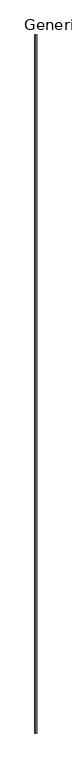
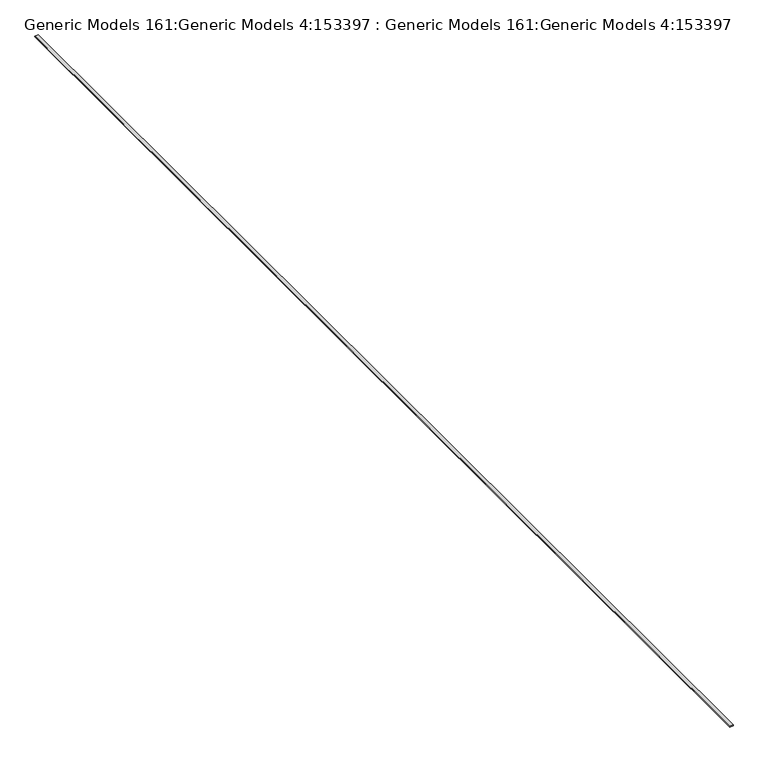
"""IFC4 building model written with IfcOpenShell, lengths in millimetres: proxy geometry, Generic Models 161:Generic Models 4:153397 : Generic Models 161:Generic Models 4:153397."""

import ifcopenshell
import ifcopenshell.guid

model = None  # the IFC model being written
_history = None  # IfcOwnerHistory: only IFC2X3 demands one
_inside = {}  # id of a spatial element -> (the spatial element, [elements in it])
_under = {}  # id of a project, library or spatial element -> (it, [spatial elements below it])
_declared = {}  # id of a project -> (the project, [libraries it declares])
_typed = {}  # id of a type object -> (the type object, [elements of that type])
_made_of = {}  # id of a material, layer set ... -> (it, [elements and type objects made of it])


def new_model(schema):
    """Start an empty IFC model of exactly this schema.

    Asked for "IFC4X3", IfcOpenShell would pick the latest addendum, in which some entities
    have other attributes; the version numbers below select the first issue.
    IFC2X3 requires an IfcOwnerHistory on every rooted entity: one is made here for all.
    """
    global model, _history
    if schema == "IFC4X3":
        model = ifcopenshell.file(schema_version=(4, 3, 0, 0))
    else:
        model = ifcopenshell.file(schema=schema)
    _inside.clear()
    _under.clear()
    _declared.clear()
    _typed.clear()
    _made_of.clear()
    _history = None
    if model.schema == "IFC2X3":
        org = make("IfcOrganization", Name="unknown")
        user = make(
            "IfcPersonAndOrganization",
            ThePerson=make("IfcPerson", FamilyName="unknown"),
            TheOrganization=org,
        )
        app = make(
            "IfcApplication",
            ApplicationDeveloper=org,
            Version="unknown",
            ApplicationFullName="unknown",
            ApplicationIdentifier="unknown",
        )
        _history = make(
            "IfcOwnerHistory",
            OwningUser=user,
            OwningApplication=app,
            ChangeAction="ADDED",
            CreationDate=0,
        )
    return model


def make(cls, **values):
    """One entity of the class cls with the attributes given. An attribute that is None is left unset."""
    return model.create_entity(
        cls, **{name: value for name, value in values.items() if value is not None}
    )


def rooted(cls, **values):
    """An entity with a GlobalId (a new one), such as an element, a storey or a relation."""
    return make(cls, GlobalId=ifcopenshell.guid.new(), OwnerHistory=_history, **values)


def si_unit(unit_type, name, prefix=None):
    """IfcSIUnit, for example si_unit("LENGTHUNIT", "METRE", prefix="MILLI")."""
    return make("IfcSIUnit", UnitType=unit_type, Prefix=prefix, Name=name)


def assignment(units):
    """IfcUnitAssignment: the units of a project."""
    return None if units is None else make("IfcUnitAssignment", Units=units)


def point(xyz):
    """IfcCartesianPoint."""
    return None if xyz is None else make("IfcCartesianPoint", Coordinates=xyz)


def direction(xyz):
    """IfcDirection."""
    return None if xyz is None else make("IfcDirection", DirectionRatios=xyz)


def frame(location, z_axis=None, x_axis=None):
    """IfcAxis2Placement3D, a coordinate frame: its origin and axes. An axis left out is left unset."""
    return make(
        "IfcAxis2Placement3D",
        Location=point(location),
        Axis=direction(z_axis),
        RefDirection=direction(x_axis),
    )


def frame_2d(location, x_axis=None):
    """IfcAxis2Placement2D, a coordinate frame in the plane: its origin and x axis."""
    return make(
        "IfcAxis2Placement2D", Location=point(location), RefDirection=direction(x_axis)
    )


def origin():
    """The frame at (0, 0, 0) with its axes left unset."""
    return frame((0.0, 0.0, 0.0))


def place(relative_to, where):
    """IfcLocalPlacement: puts the frame where relative to a parent placement (None: the world)."""
    return make(
        "IfcLocalPlacement", PlacementRelTo=relative_to, RelativePlacement=where
    )


def context(
    kind, dimensions, precision=None, world=None, true_north=None, identifier=None
):
    """IfcGeometricRepresentationContext, for example the 3D "Model" context."""
    return make(
        "IfcGeometricRepresentationContext",
        ContextIdentifier=identifier,
        ContextType=kind,
        CoordinateSpaceDimension=dimensions,
        Precision=precision,
        WorldCoordinateSystem=world,
        TrueNorth=true_north,
    )


def project(units=None, contexts=None):
    """IfcProject with its units and contexts."""
    return rooted(
        "IfcProject",
        Name="project",
        RepresentationContexts=contexts,
        UnitsInContext=assignment(units),
    )


def spatial(cls, under=None, at=None, **own):
    """A site, building, storey or space (cls), placed at a placement, below another one or the project."""
    s = rooted(cls, ObjectPlacement=at, **own)
    if under is not None:
        _under.setdefault(under.id(), (under, []))[1].append(s)
    return s


def polyline(points):
    """IfcPolyline through the points."""
    return make("IfcPolyline", Points=[point(p) for p in points])


def circle_curve(where, radius):
    """IfcCircle in the frame where."""
    return make("IfcCircle", Position=where, Radius=radius)


def trimmed(basis, trim1, trim2, sense, master):
    """IfcTrimmedCurve: the piece of a basis curve between two trims."""
    return make(
        "IfcTrimmedCurve",
        BasisCurve=basis,
        Trim1=trim1,
        Trim2=trim2,
        SenseAgreement=sense,
        MasterRepresentation=master,
    )


def segment(curve, same_sense, transition):
    """IfcCompositeCurveSegment."""
    return make(
        "IfcCompositeCurveSegment",
        Transition=transition,
        SameSense=same_sense,
        ParentCurve=curve,
    )


def composite_curve(segments, self_intersect=None):
    """IfcCompositeCurve: segments joined end to end."""
    return make("IfcCompositeCurve", Segments=segments, SelfIntersect=self_intersect)


def outline(outer, holes=None, kind="AREA"):
    """IfcArbitraryClosedProfileDef: a profile drawn as a closed curve; with holes, ...WithVoids."""
    if holes is None:
        return make("IfcArbitraryClosedProfileDef", ProfileType=kind, OuterCurve=outer)
    return make(
        "IfcArbitraryProfileDefWithVoids",
        ProfileType=kind,
        OuterCurve=outer,
        InnerCurves=holes,
    )


def extrude(swept, where, along, depth):
    """IfcExtrudedAreaSolid: the profile swept, set in the frame where, extruded along a direction by depth."""
    return make(
        "IfcExtrudedAreaSolid",
        SweptArea=swept,
        Position=where,
        ExtrudedDirection=direction(along),
        Depth=depth,
    )


def shape(context_of_items, identifier, shape_type, items):
    """IfcShapeRepresentation: the items that make up one representation, for example the "Body"."""
    return make(
        "IfcShapeRepresentation",
        ContextOfItems=context_of_items,
        RepresentationIdentifier=identifier,
        RepresentationType=shape_type,
        Items=items,
    )


def source(mapping_origin, context_of_items, identifier, shape_type, items):
    """IfcRepresentationMap: a shape defined once, which mapped items show again and again."""
    return make(
        "IfcRepresentationMap",
        MappingOrigin=mapping_origin,
        MappedRepresentation=shape(context_of_items, identifier, shape_type, items),
    )


def transform(
    local_origin,
    x_axis=None,
    y_axis=None,
    z_axis=None,
    scale=None,
    scale2=None,
    scale3=None,
    uniform=True,
):
    """IfcCartesianTransformationOperator3D, or its non-uniform kind. x_axis, y_axis, z_axis: its Axis1, 2, 3."""
    if uniform:
        return make(
            "IfcCartesianTransformationOperator3D",
            Axis1=direction(x_axis),
            Axis2=direction(y_axis),
            LocalOrigin=point(local_origin),
            Scale=scale,
            Axis3=direction(z_axis),
        )
    return make(
        "IfcCartesianTransformationOperator3DnonUniform",
        Axis1=direction(x_axis),
        Axis2=direction(y_axis),
        LocalOrigin=point(local_origin),
        Scale=scale,
        Axis3=direction(z_axis),
        Scale2=scale2,
        Scale3=scale3,
    )


def mapped(mapping_source, mapping_target):
    """IfcMappedItem: shows the shape of a source again, moved by a transform."""
    return make(
        "IfcMappedItem", MappingSource=mapping_source, MappingTarget=mapping_target
    )


def made_of(thing, what):
    """Note that an element or type object is made of a material, layer set ...; save() writes the relation."""
    if what is not None:
        _made_of.setdefault(what.id(), (what, []))[1].append(thing)
    return thing


def element(
    cls,
    number,
    at=None,
    inside=None,
    cuts=None,
    type_object=None,
    material=None,
    context=None,
    identifier="Body",
    shape_type=None,
    held_by="IfcProductDefinitionShape",
    body=None,
    shapes=None,
    **own,
):
    """One element of the class cls, such as IfcWall. Its Tag is "e" and its number.

    at: its placement. inside: the storey or other place that contains it. cuts: it is an
    opening in that element (IfcRelVoidsElement). A single representation is given by context,
    identifier, shape_type and body (its items); several are given by shapes. held_by: the class
    of the entity that holds the representations. save() writes the other relations.
    """
    e = rooted(cls, Tag="e%d" % number, ObjectPlacement=at, **own)
    if body is not None:
        shapes = [shape(context, identifier, shape_type, body)]
    if shapes is not None:
        e.Representation = make(held_by, Representations=shapes)
    if inside is not None:
        _inside.setdefault(inside.id(), (inside, []))[1].append(e)
    if cuts is not None:
        rooted(
            "IfcRelVoidsElement", RelatingBuildingElement=cuts, RelatedOpeningElement=e
        )
    if type_object is not None:
        _typed.setdefault(type_object.id(), (type_object, []))[1].append(e)
    return made_of(e, material)


def aggregate(whole, parts):
    """IfcRelAggregates: a whole, such as a stair, and the parts it consists of."""
    return rooted("IfcRelAggregates", RelatingObject=whole, RelatedObjects=parts)


def save(model, path):
    """Write the relations noted so far, then the file.

    IfcRelAggregates (storeys below a building ...), IfcRelContainedInSpatialStructure (elements
    in a storey), IfcRelDefinesByType, IfcRelAssociatesMaterial and IfcRelDeclares: one each for
    every whole, place, type object, material and project.
    """
    for whole, parts in _under.values():
        aggregate(whole, parts)
    for where, things in _inside.values():
        rooted(
            "IfcRelContainedInSpatialStructure",
            RelatedElements=things,
            RelatingStructure=where,
        )
    for kind, things in _typed.values():
        rooted("IfcRelDefinesByType", RelatedObjects=things, RelatingType=kind)
    for what, things in _made_of.values():
        rooted("IfcRelAssociatesMaterial", RelatedObjects=things, RelatingMaterial=what)
    for by, libraries in _declared.values():
        rooted("IfcRelDeclares", RelatingContext=by, RelatedDefinitions=libraries)
    model.write(path)


def generic_models_161_generic_models_4_153397_generic_models_bcc9808c(model_context):
    return source(origin(), model_context, "Body", "SweptSolid", [
        extrude(outline(composite_curve([segment(polyline([(-342.0475126, -10294.1571126), (-342.0475126, -10331.3078813)]), True, "CONTINUOUS"), segment(trimmed(circle_curve(frame_2d((-346.8100126, -10333.721994)), 5.3394144), [point((-342.0475126, -10331.3078813))], [point((-351.5725126, -10331.3078813))], True, "CARTESIAN"), True, "CONTINUOUS"), segment(polyline([(-351.5725126, -10331.3078813), (-351.5725126, -10294.1571126), (-342.0475126, -10294.1571126)]), True, "CONTINUOUS")], self_intersect=False)), frame((0.0, -5303.1974793, 0.0), z_axis=(0.0, 1.0, 0.0), x_axis=(0.0, 0.0, 1.0)), (0.0, 0.0, 1.0), 12547.6),
    ])


if __name__ == "__main__":
    model = new_model("IFC4")
    model_context = context("Model", 3, world=origin())
    ifc_project = project(units=[si_unit("LENGTHUNIT", "METRE", prefix="MILLI")], contexts=[model_context])
    site = spatial("IfcSite", under=ifc_project)
    building = spatial("IfcBuilding", under=site)
    placement = place(None, origin())
    generic_models_161_generic_models_4_153397_generic_models_shape = generic_models_161_generic_models_4_153397_generic_models_bcc9808c(model_context)
    element("IfcBuildingElementProxy", 1, Name="Generic Models 161:Generic Models 4:153397 : Generic Models 161:Generic Models 4:153397", ObjectType="Generic Models 161:Generic Models 4:153397 : Generic Models 161:Generic Models 4:153397", at=placement, inside=building, context=model_context, shape_type="MappedRepresentation", body=[
        mapped(generic_models_161_generic_models_4_153397_generic_models_shape, transform((0.0, 0.0, 0.0), x_axis=(1.0, 0.0, 0.0), y_axis=(0.0, 1.0, 0.0), z_axis=(0.0, 0.0, 1.0))),
    ])
    save(model, "model.ifc")

# Revit data of these elements
# Type "Generic Models 161:Generic Models 4:153397 : Generic Models 161:Generic Models 4:153397"
#   NameOverride = "Generic Models 161:Generic Models 4:153397"
#   ObjectTypeOverride = "Generic Models 161:Generic Models 4"
#   Reference = "Generic Models 4"
#   Category = "Generic Models"
#   Tag = "153397"
# Element 1 (IfcBuildingElementProxy, "Generic Models 161:Generic Models 4:153397 : Generic Models 161:Generic Models 4:153397")
#   Materials on its faces: "_MORTAR SETTING BED 12838"
# Materials
#   "_MORTAR SETTING BED 12838": class "Unassigned", colour RGB 191 191 191, transparency 0
